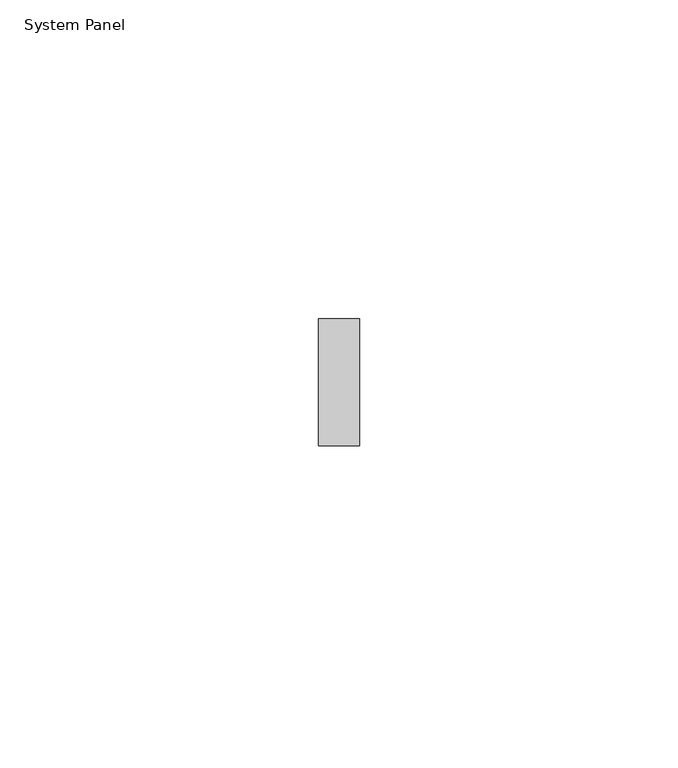
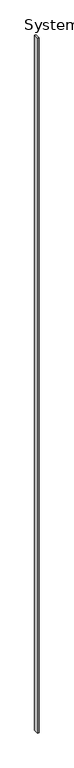
"""IFC4 building model written with IfcOpenShell, lengths in millimetres: plate geometry, System Panel : WWm-Glass-20mm-10mmOffset."""

from ifc_helpers import new_model, si_unit, origin, origin_with_axes, place, context, project, spatial, polyline, outline, extrude, source, transform, mapped, element, save


def system_panel_44d3e369(model_context):
    return source(origin(), model_context, "Body", "SweptSolid", [
        extrude(outline(polyline([(3.2340399, 0.0), (-3.2340399, 0.0), (-3.2340399, 20.0), (3.2340399, 20.0), (3.2340399, 0.0)])), origin_with_axes(), (0.0, 0.0, 1.0), 3150.0),
    ])


if __name__ == "__main__":
    model = new_model("IFC4")
    model_context = context("Model", 3, world=origin())
    ifc_project = project(units=[si_unit("LENGTHUNIT", "METRE", prefix="MILLI")], contexts=[model_context])
    site = spatial("IfcSite", under=ifc_project)
    building = spatial("IfcBuilding", under=site)
    placement = place(None, origin())
    system_panel_shape = system_panel_44d3e369(model_context)
    element("IfcPlate", 1, ObjectType="System Panel : WWm-Glass-20mm-10mmOffset", at=placement, inside=building, context=model_context, shape_type="MappedRepresentation", body=[
        mapped(system_panel_shape, transform((0.0, 0.0, 0.0), x_axis=(1.0, 0.0, 0.0), y_axis=(0.0, 1.0, 0.0), z_axis=(0.0, 0.0, 1.0))),
    ])
    save(model, "model.ifc")

# Revit data of these elements
# Type "System Panel : WWm-Glass-20mm-10mmOffset"
#   Finish = ""
# Element 1 (IfcPlate, "System Panel : WWm-Glass-20mm-10mmOffset")
#   Materials on its faces: "WW-EC-GL-Storefront"
# Materials
#   "WW-EC-GL-Storefront": class "Glass", colour RGB 236 240 239, transparency 0.85, Description = "Storefront Glass", Cost = 0
